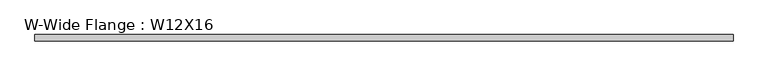
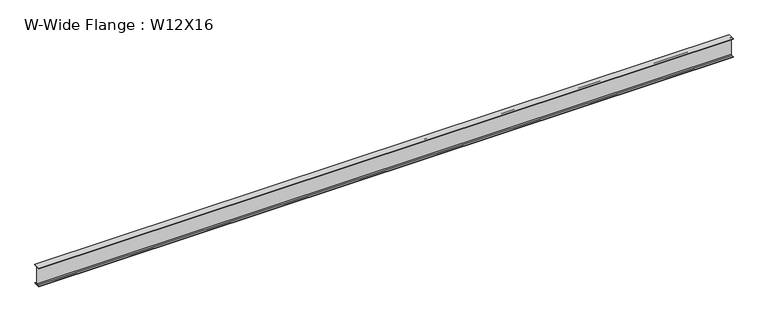
"""IFC4 building model written with IfcOpenShell, lengths in millimetres: beam geometry, W-Wide Flange : W12X16."""

import ifcopenshell
import ifcopenshell.guid

model = None  # the IFC model being written
_history = None  # IfcOwnerHistory: only IFC2X3 demands one
_inside = {}  # id of a spatial element -> (the spatial element, [elements in it])
_under = {}  # id of a project, library or spatial element -> (it, [spatial elements below it])
_declared = {}  # id of a project -> (the project, [libraries it declares])
_typed = {}  # id of a type object -> (the type object, [elements of that type])
_made_of = {}  # id of a material, layer set ... -> (it, [elements and type objects made of it])


def new_model(schema):
    """Start an empty IFC model of exactly this schema.

    Asked for "IFC4X3", IfcOpenShell would pick the latest addendum, in which some entities
    have other attributes; the version numbers below select the first issue.
    IFC2X3 requires an IfcOwnerHistory on every rooted entity: one is made here for all.
    """
    global model, _history
    if schema == "IFC4X3":
        model = ifcopenshell.file(schema_version=(4, 3, 0, 0))
    else:
        model = ifcopenshell.file(schema=schema)
    _inside.clear()
    _under.clear()
    _declared.clear()
    _typed.clear()
    _made_of.clear()
    _history = None
    if model.schema == "IFC2X3":
        org = make("IfcOrganization", Name="unknown")
        user = make(
            "IfcPersonAndOrganization",
            ThePerson=make("IfcPerson", FamilyName="unknown"),
            TheOrganization=org,
        )
        app = make(
            "IfcApplication",
            ApplicationDeveloper=org,
            Version="unknown",
            ApplicationFullName="unknown",
            ApplicationIdentifier="unknown",
        )
        _history = make(
            "IfcOwnerHistory",
            OwningUser=user,
            OwningApplication=app,
            ChangeAction="ADDED",
            CreationDate=0,
        )
    return model


def make(cls, **values):
    """One entity of the class cls with the attributes given. An attribute that is None is left unset."""
    return model.create_entity(
        cls, **{name: value for name, value in values.items() if value is not None}
    )


def rooted(cls, **values):
    """An entity with a GlobalId (a new one), such as an element, a storey or a relation."""
    return make(cls, GlobalId=ifcopenshell.guid.new(), OwnerHistory=_history, **values)


def si_unit(unit_type, name, prefix=None):
    """IfcSIUnit, for example si_unit("LENGTHUNIT", "METRE", prefix="MILLI")."""
    return make("IfcSIUnit", UnitType=unit_type, Prefix=prefix, Name=name)


def assignment(units):
    """IfcUnitAssignment: the units of a project."""
    return None if units is None else make("IfcUnitAssignment", Units=units)


def point(xyz):
    """IfcCartesianPoint."""
    return None if xyz is None else make("IfcCartesianPoint", Coordinates=xyz)


def direction(xyz):
    """IfcDirection."""
    return None if xyz is None else make("IfcDirection", DirectionRatios=xyz)


def frame(location, z_axis=None, x_axis=None):
    """IfcAxis2Placement3D, a coordinate frame: its origin and axes. An axis left out is left unset."""
    return make(
        "IfcAxis2Placement3D",
        Location=point(location),
        Axis=direction(z_axis),
        RefDirection=direction(x_axis),
    )


def frame_2d(location, x_axis=None):
    """IfcAxis2Placement2D, a coordinate frame in the plane: its origin and x axis."""
    return make(
        "IfcAxis2Placement2D", Location=point(location), RefDirection=direction(x_axis)
    )


def origin():
    """The frame at (0, 0, 0) with its axes left unset."""
    return frame((0.0, 0.0, 0.0))


def place(relative_to, where):
    """IfcLocalPlacement: puts the frame where relative to a parent placement (None: the world)."""
    return make(
        "IfcLocalPlacement", PlacementRelTo=relative_to, RelativePlacement=where
    )


def context(
    kind, dimensions, precision=None, world=None, true_north=None, identifier=None
):
    """IfcGeometricRepresentationContext, for example the 3D "Model" context."""
    return make(
        "IfcGeometricRepresentationContext",
        ContextIdentifier=identifier,
        ContextType=kind,
        CoordinateSpaceDimension=dimensions,
        Precision=precision,
        WorldCoordinateSystem=world,
        TrueNorth=true_north,
    )


def project(units=None, contexts=None):
    """IfcProject with its units and contexts."""
    return rooted(
        "IfcProject",
        Name="project",
        RepresentationContexts=contexts,
        UnitsInContext=assignment(units),
    )


def spatial(cls, under=None, at=None, **own):
    """A site, building, storey or space (cls), placed at a placement, below another one or the project."""
    s = rooted(cls, ObjectPlacement=at, **own)
    if under is not None:
        _under.setdefault(under.id(), (under, []))[1].append(s)
    return s


def polyline(points):
    """IfcPolyline through the points."""
    return make("IfcPolyline", Points=[point(p) for p in points])


def circle_curve(where, radius):
    """IfcCircle in the frame where."""
    return make("IfcCircle", Position=where, Radius=radius)


def trimmed(basis, trim1, trim2, sense, master):
    """IfcTrimmedCurve: the piece of a basis curve between two trims."""
    return make(
        "IfcTrimmedCurve",
        BasisCurve=basis,
        Trim1=trim1,
        Trim2=trim2,
        SenseAgreement=sense,
        MasterRepresentation=master,
    )


def segment(curve, same_sense, transition):
    """IfcCompositeCurveSegment."""
    return make(
        "IfcCompositeCurveSegment",
        Transition=transition,
        SameSense=same_sense,
        ParentCurve=curve,
    )


def composite_curve(segments, self_intersect=None):
    """IfcCompositeCurve: segments joined end to end."""
    return make("IfcCompositeCurve", Segments=segments, SelfIntersect=self_intersect)


def outline(outer, holes=None, kind="AREA"):
    """IfcArbitraryClosedProfileDef: a profile drawn as a closed curve; with holes, ...WithVoids."""
    if holes is None:
        return make("IfcArbitraryClosedProfileDef", ProfileType=kind, OuterCurve=outer)
    return make(
        "IfcArbitraryProfileDefWithVoids",
        ProfileType=kind,
        OuterCurve=outer,
        InnerCurves=holes,
    )


def extrude(swept, where, along, depth):
    """IfcExtrudedAreaSolid: the profile swept, set in the frame where, extruded along a direction by depth."""
    return make(
        "IfcExtrudedAreaSolid",
        SweptArea=swept,
        Position=where,
        ExtrudedDirection=direction(along),
        Depth=depth,
    )


def shape(context_of_items, identifier, shape_type, items):
    """IfcShapeRepresentation: the items that make up one representation, for example the "Body"."""
    return make(
        "IfcShapeRepresentation",
        ContextOfItems=context_of_items,
        RepresentationIdentifier=identifier,
        RepresentationType=shape_type,
        Items=items,
    )


def source(mapping_origin, context_of_items, identifier, shape_type, items):
    """IfcRepresentationMap: a shape defined once, which mapped items show again and again."""
    return make(
        "IfcRepresentationMap",
        MappingOrigin=mapping_origin,
        MappedRepresentation=shape(context_of_items, identifier, shape_type, items),
    )


def transform(
    local_origin,
    x_axis=None,
    y_axis=None,
    z_axis=None,
    scale=None,
    scale2=None,
    scale3=None,
    uniform=True,
):
    """IfcCartesianTransformationOperator3D, or its non-uniform kind. x_axis, y_axis, z_axis: its Axis1, 2, 3."""
    if uniform:
        return make(
            "IfcCartesianTransformationOperator3D",
            Axis1=direction(x_axis),
            Axis2=direction(y_axis),
            LocalOrigin=point(local_origin),
            Scale=scale,
            Axis3=direction(z_axis),
        )
    return make(
        "IfcCartesianTransformationOperator3DnonUniform",
        Axis1=direction(x_axis),
        Axis2=direction(y_axis),
        LocalOrigin=point(local_origin),
        Scale=scale,
        Axis3=direction(z_axis),
        Scale2=scale2,
        Scale3=scale3,
    )


def mapped(mapping_source, mapping_target):
    """IfcMappedItem: shows the shape of a source again, moved by a transform."""
    return make(
        "IfcMappedItem", MappingSource=mapping_source, MappingTarget=mapping_target
    )


def made_of(thing, what):
    """Note that an element or type object is made of a material, layer set ...; save() writes the relation."""
    if what is not None:
        _made_of.setdefault(what.id(), (what, []))[1].append(thing)
    return thing


def element(
    cls,
    number,
    at=None,
    inside=None,
    cuts=None,
    type_object=None,
    material=None,
    context=None,
    identifier="Body",
    shape_type=None,
    held_by="IfcProductDefinitionShape",
    body=None,
    shapes=None,
    **own,
):
    """One element of the class cls, such as IfcWall. Its Tag is "e" and its number.

    at: its placement. inside: the storey or other place that contains it. cuts: it is an
    opening in that element (IfcRelVoidsElement). A single representation is given by context,
    identifier, shape_type and body (its items); several are given by shapes. held_by: the class
    of the entity that holds the representations. save() writes the other relations.
    """
    e = rooted(cls, Tag="e%d" % number, ObjectPlacement=at, **own)
    if body is not None:
        shapes = [shape(context, identifier, shape_type, body)]
    if shapes is not None:
        e.Representation = make(held_by, Representations=shapes)
    if inside is not None:
        _inside.setdefault(inside.id(), (inside, []))[1].append(e)
    if cuts is not None:
        rooted(
            "IfcRelVoidsElement", RelatingBuildingElement=cuts, RelatedOpeningElement=e
        )
    if type_object is not None:
        _typed.setdefault(type_object.id(), (type_object, []))[1].append(e)
    return made_of(e, material)


def aggregate(whole, parts):
    """IfcRelAggregates: a whole, such as a stair, and the parts it consists of."""
    return rooted("IfcRelAggregates", RelatingObject=whole, RelatedObjects=parts)


def save(model, path):
    """Write the relations noted so far, then the file.

    IfcRelAggregates (storeys below a building ...), IfcRelContainedInSpatialStructure (elements
    in a storey), IfcRelDefinesByType, IfcRelAssociatesMaterial and IfcRelDeclares: one each for
    every whole, place, type object, material and project.
    """
    for whole, parts in _under.values():
        aggregate(whole, parts)
    for where, things in _inside.values():
        rooted(
            "IfcRelContainedInSpatialStructure",
            RelatedElements=things,
            RelatingStructure=where,
        )
    for kind, things in _typed.values():
        rooted("IfcRelDefinesByType", RelatedObjects=things, RelatingType=kind)
    for what, things in _made_of.values():
        rooted("IfcRelAssociatesMaterial", RelatedObjects=things, RelatingMaterial=what)
    for by, libraries in _declared.values():
        rooted("IfcRelDeclares", RelatingContext=by, RelatedDefinitions=libraries)
    model.write(path)


def w_wide_flange_w12x16_17ea960c(model_context):
    return source(origin(), model_context, "Body", "SweptSolid", [
        extrude(outline(composite_curve([segment(polyline([(50.673, -145.669), (50.673, -152.4), (-50.673, -152.4), (-50.673, -145.669), (-16.7005, -145.669)]), True, "CONTINUOUS"), segment(trimmed(circle_curve(frame_2d((-16.7005, -131.7625)), 13.9065), [point((-16.7005, -145.669))], [point((-2.794, -131.7625))], True, "CARTESIAN"), True, "CONTINUOUS"), segment(polyline([(-2.794, -131.7625), (-2.794, 131.7625)]), True, "CONTINUOUS"), segment(trimmed(circle_curve(frame_2d((-16.7005, 131.7625)), 13.9065), [point((-2.794, 131.7625))], [point((-16.7005, 145.669))], True, "CARTESIAN"), True, "CONTINUOUS"), segment(polyline([(-16.7005, 145.669), (-50.673, 145.669), (-50.673, 152.4), (50.673, 152.4), (50.673, 145.669), (16.7005, 145.669)]), True, "CONTINUOUS"), segment(trimmed(circle_curve(frame_2d((16.7005, 131.7625)), 13.9065), [point((16.7005, 145.669))], [point((2.794, 131.7625))], True, "CARTESIAN"), True, "CONTINUOUS"), segment(polyline([(2.794, 131.7625), (2.794, -131.7625)]), True, "CONTINUOUS"), segment(trimmed(circle_curve(frame_2d((16.7005, -131.7625)), 13.9065), [point((2.794, -131.7625))], [point((16.7005, -145.669))], True, "CARTESIAN"), True, "CONTINUOUS"), segment(polyline([(16.7005, -145.669), (50.673, -145.669)]), True, "CONTINUOUS")], self_intersect=False)), frame((-5393.7497188, 0.0, 0.0), z_axis=(1.0, 0.0, 0.0), x_axis=(0.0, 1.0, 0.0)), (0.0, 0.0, 1.0), 10787.4994376),
    ])


if __name__ == "__main__":
    model = new_model("IFC4")
    model_context = context("Model", 3, world=origin())
    ifc_project = project(units=[si_unit("LENGTHUNIT", "METRE", prefix="MILLI")], contexts=[model_context])
    site = spatial("IfcSite", under=ifc_project)
    building = spatial("IfcBuilding", under=site)
    placement = place(None, origin())
    w_wide_flange_w12x16_shape = w_wide_flange_w12x16_17ea960c(model_context)
    element("IfcBeam", 1, ObjectType="W-Wide Flange : W12X16", at=placement, inside=building, context=model_context, shape_type="MappedRepresentation", body=[
        mapped(w_wide_flange_w12x16_shape, transform((0.0, 0.0, 0.0), x_axis=(1.0, 0.0, 0.0), y_axis=(0.0, 1.0, 0.0), z_axis=(0.0, 0.0, 1.0))),
    ])
    save(model, "model.ifc")

# Revit data of these elements
# Type "W-Wide Flange : W12X16"
#   Assembly Code = "B10"
#   W = 16
#   Length [instance default] = 5' - 0"
#   bf = 0' - 3.99"
#   d = 1' - 0"
#   k = 0' - 0 13/16"
#   k2 = 0' - 0.5475"
#   tf = 0' - 0.265"
#   tw = 0' - 0.22"
#   A = 0.0327083 SF
#   Structural Material [instance default] = Steel ASTM A992
# Element 1 (IfcBeam, "W-Wide Flange : W12X16")
#   Structural Material = STRUCTURAL STEEL - SEE STRUCT. DWGS
#   Materials on its faces: "STRUCTURAL STEEL - SEE STRUCT. DWGS"
# Materials
#   "Steel ASTM A992": class "Metal", colour RGB 199 199 199, transparency 0, Description = "Structural steel 50ksi", Cost = 0
#   "STRUCTURAL STEEL - SEE STRUCT. DWGS": class "Metal", colour RGB 137 146 153, transparency 0, Description = "Steel, mill finish", Cost = 0
